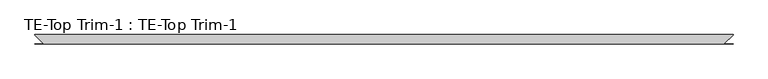
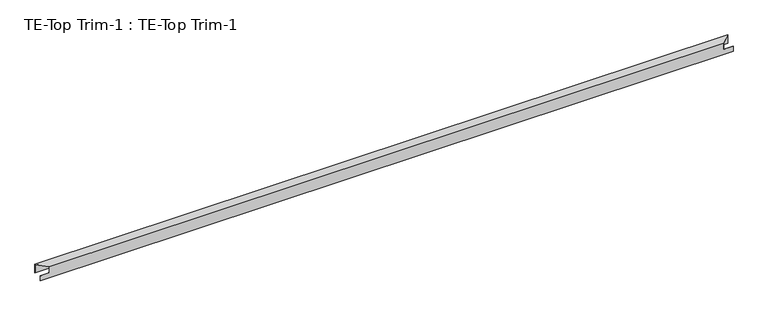
"""IFC4 building model written with IfcOpenShell, lengths in millimetres: proxy geometry, TE-Top Trim-1 : TE-Top Trim-1."""

from ifc_helpers import new_model, si_unit, origin, place, context, project, spatial, faceted_brep, source, transform, mapped, element, save


def te_top_trim_1_te_top_trim_1_ce3f5671(model_context):
    return source(origin(), model_context, "Body", "Brep", [
        faceted_brep([(587327.7934739, -531640.1093528, 2387.6), (587327.7934739, -531641.0023216, 2387.6), (587327.7934739, -531641.0023216, 2411.4125), (587327.7934739, -531640.1093528, 2411.4125), (587327.7934739, -531599.3917241, 2439.2929688), (587327.7934739, -531599.3917241, 2400.3), (587327.7934739, -531600.3289841, 2400.3), (587327.7934739, -531600.3289841, 2438.4), (587327.7934739, -531601.1251169, 2438.4), (587327.7934739, -531601.1251169, 2439.2929688), (590392.4558739, -531600.3289841, 2400.3), (590392.4558739, -531599.3917241, 2400.3), (590392.4558739, -531599.3917241, 2439.2929688), (590392.4558739, -531600.3190424, 2439.2929688), (590392.4558739, -531600.3190424, 2438.4), (590392.4558739, -531600.3289841, 2411.4125), (590392.4558739, -531641.0023216, 2387.6), (590392.4558739, -531640.1093528, 2387.6), (590392.4558739, -531640.1093528, 2411.4125), (590392.4558739, -531641.0023216, 2411.4125), (590351.7725947, -531641.0023216, 2411.4125), (590351.7725947, -531641.0023216, 2439.2929688), (587367.6706786, -531641.0023216, 2439.2929688), (587367.6706786, -531641.0023216, 2411.4125), (590352.6655635, -531640.1093528, 2438.4), (587366.7777099, -531640.1093528, 2438.4), (587366.7777099, -531640.1093528, 2411.4125), (590352.6655635, -531640.1093528, 2411.4125)], [[[0, 1, 2, 3]], [[4, 5, 6, 7, 8, 9]], [[10, 11, 12, 13, 14, 15]], [[16, 17, 18, 19]], [[1, 0, 17, 16]], [[1, 16, 19, 20, 21, 22, 23, 2]], [[12, 4, 9, 22, 21, 13]], [[5, 4, 12, 11]], [[6, 5, 11, 10]], [[7, 6, 10, 15, 14]], [[7, 14, 24, 25, 8]], [[17, 0, 3, 26, 25, 24, 27, 18]], [[27, 20, 19, 18]], [[20, 27, 24, 14, 13, 21]], [[23, 26, 3, 2]], [[26, 23, 22, 9, 8, 25]]]),
    ])


if __name__ == "__main__":
    model = new_model("IFC4")
    model_context = context("Model", 3, world=origin())
    ifc_project = project(units=[si_unit("LENGTHUNIT", "METRE", prefix="MILLI")], contexts=[model_context])
    site = spatial("IfcSite", under=ifc_project)
    building = spatial("IfcBuilding", under=site)
    placement = place(None, origin())
    te_top_trim_1_te_top_trim_1_shape = te_top_trim_1_te_top_trim_1_ce3f5671(model_context)
    element("IfcBuildingElementProxy", 1, Name="TE-Top Trim-1 : TE-Top Trim-1", ObjectType="TE-Top Trim-1 : TE-Top Trim-1", at=placement, inside=building, context=model_context, shape_type="MappedRepresentation", body=[
        mapped(te_top_trim_1_te_top_trim_1_shape, transform((0.0, 0.0, 0.0), x_axis=(1.0, 0.0, 0.0), y_axis=(0.0, 1.0, 0.0), z_axis=(0.0, 0.0, 1.0))),
    ])
    save(model, "model.ifc")

# Revit data of these elements
# Element 1 (IfcBuildingElementProxy, "TE-Top Trim-1 : TE-Top Trim-1")
#   Materials on its faces: "EDGE TRIM BY MTL PANEL MFR."
# Materials
#   "EDGE TRIM BY MTL PANEL MFR.": class "Generic", colour RGB 239 242 240, transparency 0, Cost = 0
